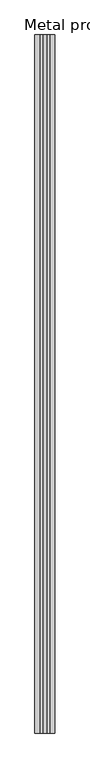
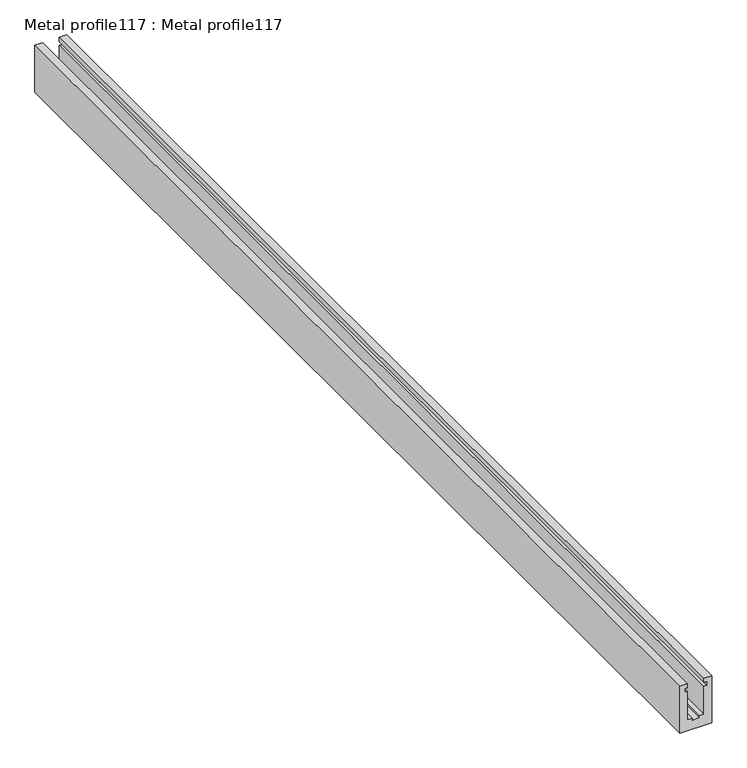
"""IFC4 building model written with IfcOpenShell, lengths in millimetres: proxy geometry, Metal profile117 : Metal profile117."""

from ifc_helpers import new_model, si_unit, frame, origin, place, context, project, spatial, polyline, outline, extrude, source, transform, mapped, element, save


def metal_profile117_metal_profile117_b841d572(model_context):
    return source(origin(), model_context, "Body", "SweptSolid", [
        extrude(outline(polyline([(40207.2092895, -7043.9834918), (40207.2092895, -7057.8334674), (40198.9413208, -7057.8334674), (40198.9413208, -7053.304964), (40192.2147583, -7053.304964), (40192.2147583, -7057.8334674), (40138.9092895, -7057.8334674), (40138.9092895, -7066.2334918), (40135.1384674, -7066.2334918), (40135.1384674, -7078.9334918), (40138.9092895, -7078.9334918), (40138.9092895, -7087.3335162), (40192.2147583, -7087.3335162), (40192.2147583, -7091.8620197), (40198.9413208, -7091.8620197), (40198.9413208, -7087.3335162), (40207.2092895, -7087.3335162), (40207.2092895, -7101.1834918), (40118.3092895, -7101.1834918), (40118.3092895, -7043.9834918), (40207.2092895, -7043.9834918)])), frame((0.0, 7182.1531721, 0.0), z_axis=(0.0, 1.0, 0.0), x_axis=(0.0, 0.0, 1.0)), (0.0, 0.0, 1.0), 1999.85),
    ])


if __name__ == "__main__":
    model = new_model("IFC4")
    model_context = context("Model", 3, world=origin())
    ifc_project = project(units=[si_unit("LENGTHUNIT", "METRE", prefix="MILLI")], contexts=[model_context])
    site = spatial("IfcSite", under=ifc_project)
    building = spatial("IfcBuilding", under=site)
    placement = place(None, origin())
    metal_profile117_metal_profile117_shape = metal_profile117_metal_profile117_b841d572(model_context)
    element("IfcBuildingElementProxy", 1, Name="Metal profile117 : Metal profile117", ObjectType="Metal profile117 : Metal profile117", at=placement, inside=building, context=model_context, shape_type="MappedRepresentation", body=[
        mapped(metal_profile117_metal_profile117_shape, transform((0.0, 0.0, 0.0), x_axis=(1.0, 0.0, 0.0), y_axis=(0.0, 1.0, 0.0), z_axis=(0.0, 0.0, 1.0))),
    ])
    save(model, "model.ifc")

# Revit data of these elements
# Type "Metal profile117 : Metal profile117"
#   NameOverride = "Metal profile117"
# Element 1 (IfcBuildingElementProxy, "Metal profile117 : Metal profile117")
#   Materials on its faces: "CR LAURENCE ALUMINIUM B5S SERIES STANDARD SQUARE BASE SHOE FOR 1/2\" TEMPERED GLASS - SEE STRUCT. DWGS"
# Materials
#   "CR LAURENCE ALUMINIUM B5S SERIES STANDARD SQUARE BASE SHOE FOR 1/2\" TEMPERED GLASS - SEE STRUCT. DWGS": class "Unassigned", colour RGB 128 128 128, transparency 0, Cost = 0
